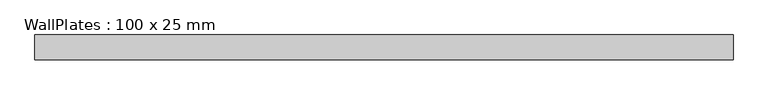
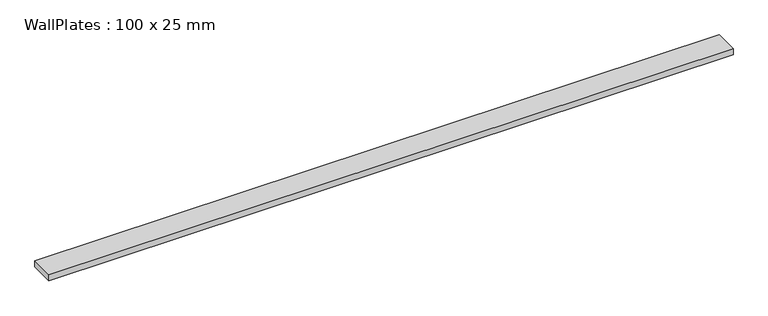
"""IFC4 building model written with IfcOpenShell, lengths in millimetres: beam geometry, WallPlates : 100 x 25 mm."""

from ifc_helpers import new_model, si_unit, frame, origin, place, context, project, spatial, polyline, outline, extrude, source, transform, mapped, element, save


def wallplates_100_x_25_mm_9696bd37(model_context):
    return source(origin(), model_context, "Body", "SweptSolid", [
        extrude(outline(polyline([(-1407.3141175, -50.0), (-1407.3141175, 50.0), (1407.3141175, 50.0), (1407.3141175, -50.0), (-1407.3141175, -50.0)])), frame((0.0, 0.0, -12.5), z_axis=(0.0, 0.0, 1.0), x_axis=(1.0, 0.0, 0.0)), (0.0, 0.0, 1.0), 25.0),
    ])


if __name__ == "__main__":
    model = new_model("IFC4")
    model_context = context("Model", 3, world=origin())
    ifc_project = project(units=[si_unit("LENGTHUNIT", "METRE", prefix="MILLI")], contexts=[model_context])
    site = spatial("IfcSite", under=ifc_project)
    building = spatial("IfcBuilding", under=site)
    placement = place(None, origin())
    wallplates_100_x_25_mm_shape = wallplates_100_x_25_mm_9696bd37(model_context)
    element("IfcBeam", 1, ObjectType="WallPlates : 100 x 25 mm", at=placement, inside=building, context=model_context, shape_type="MappedRepresentation", body=[
        mapped(wallplates_100_x_25_mm_shape, transform((0.0, 0.0, 0.0), x_axis=(1.0, 0.0, 0.0), y_axis=(0.0, 1.0, 0.0), z_axis=(0.0, 0.0, 1.0))),
    ])
    save(model, "model.ifc")

# Revit data of these elements
# Type "WallPlates : 100 x 25 mm"
#   ExpertTruss = "Height\th\r\nWidth\tb"
#   Name [instance default] = ""
#   m [instance default] = 0 mm
#   ip_c_cut [instance default] = 1025 mm
#   h_fix [instance default] = 75 mm
#   d/2 [instance default] = 1750 mm
#   c_cut_incl [instance default] = -1000 mm
#   c_cut [instance default] = 0 mm
#   alfaMax [instance default] = 0.00°
#   alfa0_2 [instance default] = 90.00°
#   Alfa_str [instance default] = 0.00°
#   Alfa_cut [instance default] = 90.00°
#   AlfaMAX [instance default] = 0.00°
#   Alfa2_0 [instance default] = 0.00°
#   Alfa2 [instance default] = 0.00°
#   Alfa1_0 [instance default] = 0.00°
#   Alfa1 [instance default] = 0.00°
#   A_max_Str [instance default] = 0.00°
#   h_void [instance default] = 25 mm
#   beam_L_0 [instance default] = 100 mm
#   beam_L [instance default] = 0 mm
#   b_void [instance default] = 110 mm
#   alfa0_1 [instance default] = 90.00°
#   b = 100 mm
#   YOffsetStr [instance default] = 0 mm
#   YOffsetEnd [instance default] = 0 mm
#   XOffsetStr_0 [instance default] = 3500 mm
#   XOffsetStr [instance default] = 0 mm
#   XOffsetEnd_0 [instance default] = 3500 mm
#   XOffsetEnd [instance default] = 0 mm
#   L_void_0 [instance default] = 100 mm
#   L_void [instance default] = 0 mm
#   E2 [instance default] = 0.00°
#   E1 [instance default] = 0.00°
#   Length [instance default] = 3500 mm
#   h = 25 mm
#   Alfa [instance default] = 0.00°
#   A_max_End [instance default] = 0.00°
#   A_max [instance default] = 0.00°
#   A4 [instance default] = 0.00°
#   A3 [instance default] = 0.00°
#   A2 [instance default] = 0.00°
#   A1 [instance default] = 0.00°
#   Material [instance default] = Wood Standard
# Element 1 (IfcBeam, "WallPlates : 100 x 25 mm")
#   d/2 = 1407.314 mm
#   XOffsetStr_0 = 2814.628 mm
#   XOffsetEnd_0 = 2814.628 mm
#   Materials on its faces: "Wood Standard"
# Materials
#   "Wood Standard": class "Drewno", colour RGB 196 146 67, transparency 0, Cost = 0
